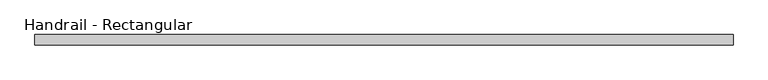
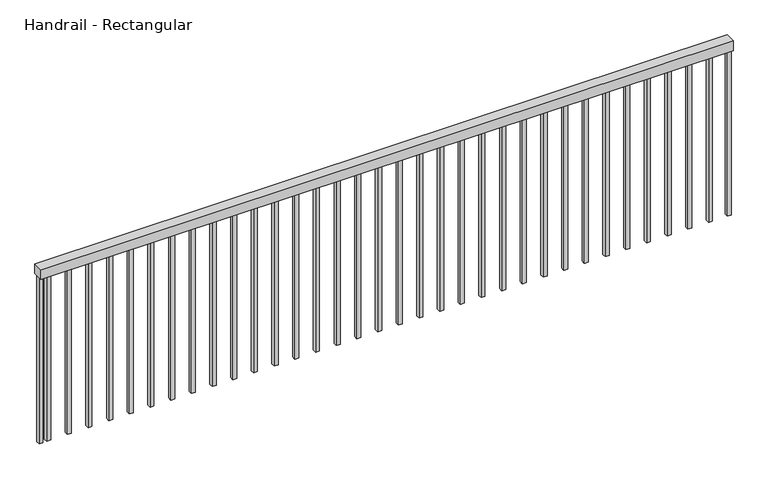
"""IFC4 building model written with IfcOpenShell, lengths in millimetres: railing geometry, Handrail - Rectangular."""

from ifc_helpers import new_model, si_unit, frame, origin, place, context, project, spatial, polyline, outline, extrude, source, transform, mapped, element, save


def handrail_rectangular_9be391eb(model_context):
    return source(origin(), model_context, "Body", "SweptSolid", [
        extrude(outline(polyline([(-6390.3046217, -592.5812264), (-6390.3046217, -643.3812264), (-9790.3046217, -643.3812264), (-9790.3046217, -592.5812264), (-6390.3046217, -592.5812264)])), frame((0.0, 0.0, 6654.4), z_axis=(0.0, 0.0, 1.0), x_axis=(1.0, 0.0, 0.0)), (0.0, 0.0, 1.0), 50.8),
        extrude(outline(polyline([(-9733.5796217, -608.4562264), (-9733.5796217, -627.5062264), (-9752.6296217, -627.5062264), (-9752.6296217, -608.4562264), (-9733.5796217, -608.4562264)])), frame((0.0, 0.0, 5790.8), z_axis=(0.0, 0.0, 1.0), x_axis=(1.0, 0.0, 0.0)), (0.0, 0.0, 1.0), 863.6),
        extrude(outline(polyline([(-9631.9796217, -608.4562264), (-9631.9796217, -627.5062264), (-9651.0296217, -627.5062264), (-9651.0296217, -608.4562264), (-9631.9796217, -608.4562264)])), frame((0.0, 0.0, 5790.8), z_axis=(0.0, 0.0, 1.0), x_axis=(1.0, 0.0, 0.0)), (0.0, 0.0, 1.0), 863.6),
        extrude(outline(polyline([(-9530.3796217, -608.4562264), (-9530.3796217, -627.5062264), (-9549.4296217, -627.5062264), (-9549.4296217, -608.4562264), (-9530.3796217, -608.4562264)])), frame((0.0, 0.0, 5790.8), z_axis=(0.0, 0.0, 1.0), x_axis=(1.0, 0.0, 0.0)), (0.0, 0.0, 1.0), 863.6),
        extrude(outline(polyline([(-9428.7796217, -608.4562264), (-9428.7796217, -627.5062264), (-9447.8296217, -627.5062264), (-9447.8296217, -608.4562264), (-9428.7796217, -608.4562264)])), frame((0.0, 0.0, 5790.8), z_axis=(0.0, 0.0, 1.0), x_axis=(1.0, 0.0, 0.0)), (0.0, 0.0, 1.0), 863.6),
        extrude(outline(polyline([(-9327.1796217, -608.4562264), (-9327.1796217, -627.5062264), (-9346.2296217, -627.5062264), (-9346.2296217, -608.4562264), (-9327.1796217, -608.4562264)])), frame((0.0, 0.0, 5790.8), z_axis=(0.0, 0.0, 1.0), x_axis=(1.0, 0.0, 0.0)), (0.0, 0.0, 1.0), 863.6),
        extrude(outline(polyline([(-9225.5796217, -608.4562264), (-9225.5796217, -627.5062264), (-9244.6296217, -627.5062264), (-9244.6296217, -608.4562264), (-9225.5796217, -608.4562264)])), frame((0.0, 0.0, 5790.8), z_axis=(0.0, 0.0, 1.0), x_axis=(1.0, 0.0, 0.0)), (0.0, 0.0, 1.0), 863.6),
        extrude(outline(polyline([(-9123.9796217, -608.4562264), (-9123.9796217, -627.5062264), (-9143.0296217, -627.5062264), (-9143.0296217, -608.4562264), (-9123.9796217, -608.4562264)])), frame((0.0, 0.0, 5790.8), z_axis=(0.0, 0.0, 1.0), x_axis=(1.0, 0.0, 0.0)), (0.0, 0.0, 1.0), 863.6),
        extrude(outline(polyline([(-9022.3796217, -608.4562264), (-9022.3796217, -627.5062264), (-9041.4296217, -627.5062264), (-9041.4296217, -608.4562264), (-9022.3796217, -608.4562264)])), frame((0.0, 0.0, 5790.8), z_axis=(0.0, 0.0, 1.0), x_axis=(1.0, 0.0, 0.0)), (0.0, 0.0, 1.0), 863.6),
        extrude(outline(polyline([(-8920.7796217, -608.4562264), (-8920.7796217, -627.5062264), (-8939.8296217, -627.5062264), (-8939.8296217, -608.4562264), (-8920.7796217, -608.4562264)])), frame((0.0, 0.0, 5790.8), z_axis=(0.0, 0.0, 1.0), x_axis=(1.0, 0.0, 0.0)), (0.0, 0.0, 1.0), 863.6),
        extrude(outline(polyline([(-8819.1796217, -608.4562264), (-8819.1796217, -627.5062264), (-8838.2296217, -627.5062264), (-8838.2296217, -608.4562264), (-8819.1796217, -608.4562264)])), frame((0.0, 0.0, 5790.8), z_axis=(0.0, 0.0, 1.0), x_axis=(1.0, 0.0, 0.0)), (0.0, 0.0, 1.0), 863.6),
        extrude(outline(polyline([(-8717.5796217, -608.4562264), (-8717.5796217, -627.5062264), (-8736.6296217, -627.5062264), (-8736.6296217, -608.4562264), (-8717.5796217, -608.4562264)])), frame((0.0, 0.0, 5790.8), z_axis=(0.0, 0.0, 1.0), x_axis=(1.0, 0.0, 0.0)), (0.0, 0.0, 1.0), 863.6),
        extrude(outline(polyline([(-8615.9796217, -608.4562264), (-8615.9796217, -627.5062264), (-8635.0296217, -627.5062264), (-8635.0296217, -608.4562264), (-8615.9796217, -608.4562264)])), frame((0.0, 0.0, 5790.8), z_axis=(0.0, 0.0, 1.0), x_axis=(1.0, 0.0, 0.0)), (0.0, 0.0, 1.0), 863.6),
        extrude(outline(polyline([(-8514.3796217, -608.4562264), (-8514.3796217, -627.5062264), (-8533.4296217, -627.5062264), (-8533.4296217, -608.4562264), (-8514.3796217, -608.4562264)])), frame((0.0, 0.0, 5790.8), z_axis=(0.0, 0.0, 1.0), x_axis=(1.0, 0.0, 0.0)), (0.0, 0.0, 1.0), 863.6),
        extrude(outline(polyline([(-8412.7796217, -608.4562264), (-8412.7796217, -627.5062264), (-8431.8296217, -627.5062264), (-8431.8296217, -608.4562264), (-8412.7796217, -608.4562264)])), frame((0.0, 0.0, 5790.8), z_axis=(0.0, 0.0, 1.0), x_axis=(1.0, 0.0, 0.0)), (0.0, 0.0, 1.0), 863.6),
        extrude(outline(polyline([(-8311.1796217, -608.4562264), (-8311.1796217, -627.5062264), (-8330.2296217, -627.5062264), (-8330.2296217, -608.4562264), (-8311.1796217, -608.4562264)])), frame((0.0, 0.0, 5790.8), z_axis=(0.0, 0.0, 1.0), x_axis=(1.0, 0.0, 0.0)), (0.0, 0.0, 1.0), 863.6),
        extrude(outline(polyline([(-8209.5796217, -608.4562264), (-8209.5796217, -627.5062264), (-8228.6296217, -627.5062264), (-8228.6296217, -608.4562264), (-8209.5796217, -608.4562264)])), frame((0.0, 0.0, 5790.8), z_axis=(0.0, 0.0, 1.0), x_axis=(1.0, 0.0, 0.0)), (0.0, 0.0, 1.0), 863.6),
        extrude(outline(polyline([(-8107.9796217, -608.4562264), (-8107.9796217, -627.5062264), (-8127.0296217, -627.5062264), (-8127.0296217, -608.4562264), (-8107.9796217, -608.4562264)])), frame((0.0, 0.0, 5790.8), z_axis=(0.0, 0.0, 1.0), x_axis=(1.0, 0.0, 0.0)), (0.0, 0.0, 1.0), 863.6),
        extrude(outline(polyline([(-8006.3796217, -608.4562264), (-8006.3796217, -627.5062264), (-8025.4296217, -627.5062264), (-8025.4296217, -608.4562264), (-8006.3796217, -608.4562264)])), frame((0.0, 0.0, 5790.8), z_axis=(0.0, 0.0, 1.0), x_axis=(1.0, 0.0, 0.0)), (0.0, 0.0, 1.0), 863.6),
        extrude(outline(polyline([(-7904.7796217, -608.4562264), (-7904.7796217, -627.5062264), (-7923.8296217, -627.5062264), (-7923.8296217, -608.4562264), (-7904.7796217, -608.4562264)])), frame((0.0, 0.0, 5790.8), z_axis=(0.0, 0.0, 1.0), x_axis=(1.0, 0.0, 0.0)), (0.0, 0.0, 1.0), 863.6),
        extrude(outline(polyline([(-7803.1796217, -608.4562264), (-7803.1796217, -627.5062264), (-7822.2296217, -627.5062264), (-7822.2296217, -608.4562264), (-7803.1796217, -608.4562264)])), frame((0.0, 0.0, 5790.8), z_axis=(0.0, 0.0, 1.0), x_axis=(1.0, 0.0, 0.0)), (0.0, 0.0, 1.0), 863.6),
        extrude(outline(polyline([(-7701.5796217, -608.4562264), (-7701.5796217, -627.5062264), (-7720.6296217, -627.5062264), (-7720.6296217, -608.4562264), (-7701.5796217, -608.4562264)])), frame((0.0, 0.0, 5790.8), z_axis=(0.0, 0.0, 1.0), x_axis=(1.0, 0.0, 0.0)), (0.0, 0.0, 1.0), 863.6),
        extrude(outline(polyline([(-7599.9796217, -608.4562264), (-7599.9796217, -627.5062264), (-7619.0296217, -627.5062264), (-7619.0296217, -608.4562264), (-7599.9796217, -608.4562264)])), frame((0.0, 0.0, 5790.8), z_axis=(0.0, 0.0, 1.0), x_axis=(1.0, 0.0, 0.0)), (0.0, 0.0, 1.0), 863.6),
        extrude(outline(polyline([(-7498.3796217, -608.4562264), (-7498.3796217, -627.5062264), (-7517.4296217, -627.5062264), (-7517.4296217, -608.4562264), (-7498.3796217, -608.4562264)])), frame((0.0, 0.0, 5790.8), z_axis=(0.0, 0.0, 1.0), x_axis=(1.0, 0.0, 0.0)), (0.0, 0.0, 1.0), 863.6),
        extrude(outline(polyline([(-7396.7796217, -608.4562264), (-7396.7796217, -627.5062264), (-7415.8296217, -627.5062264), (-7415.8296217, -608.4562264), (-7396.7796217, -608.4562264)])), frame((0.0, 0.0, 5790.8), z_axis=(0.0, 0.0, 1.0), x_axis=(1.0, 0.0, 0.0)), (0.0, 0.0, 1.0), 863.6),
        extrude(outline(polyline([(-7295.1796217, -608.4562264), (-7295.1796217, -627.5062264), (-7314.2296217, -627.5062264), (-7314.2296217, -608.4562264), (-7295.1796217, -608.4562264)])), frame((0.0, 0.0, 5790.8), z_axis=(0.0, 0.0, 1.0), x_axis=(1.0, 0.0, 0.0)), (0.0, 0.0, 1.0), 863.6),
        extrude(outline(polyline([(-7193.5796217, -608.4562264), (-7193.5796217, -627.5062264), (-7212.6296217, -627.5062264), (-7212.6296217, -608.4562264), (-7193.5796217, -608.4562264)])), frame((0.0, 0.0, 5790.8), z_axis=(0.0, 0.0, 1.0), x_axis=(1.0, 0.0, 0.0)), (0.0, 0.0, 1.0), 863.6),
        extrude(outline(polyline([(-7091.9796217, -608.4562264), (-7091.9796217, -627.5062264), (-7111.0296217, -627.5062264), (-7111.0296217, -608.4562264), (-7091.9796217, -608.4562264)])), frame((0.0, 0.0, 5790.8), z_axis=(0.0, 0.0, 1.0), x_axis=(1.0, 0.0, 0.0)), (0.0, 0.0, 1.0), 863.6),
        extrude(outline(polyline([(-6990.3796217, -608.4562264), (-6990.3796217, -627.5062264), (-7009.4296217, -627.5062264), (-7009.4296217, -608.4562264), (-6990.3796217, -608.4562264)])), frame((0.0, 0.0, 5790.8), z_axis=(0.0, 0.0, 1.0), x_axis=(1.0, 0.0, 0.0)), (0.0, 0.0, 1.0), 863.6),
        extrude(outline(polyline([(-6888.7796217, -608.4562264), (-6888.7796217, -627.5062264), (-6907.8296217, -627.5062264), (-6907.8296217, -608.4562264), (-6888.7796217, -608.4562264)])), frame((0.0, 0.0, 5790.8), z_axis=(0.0, 0.0, 1.0), x_axis=(1.0, 0.0, 0.0)), (0.0, 0.0, 1.0), 863.6),
        extrude(outline(polyline([(-6787.1796217, -608.4562264), (-6787.1796217, -627.5062264), (-6806.2296217, -627.5062264), (-6806.2296217, -608.4562264), (-6787.1796217, -608.4562264)])), frame((0.0, 0.0, 5790.8), z_axis=(0.0, 0.0, 1.0), x_axis=(1.0, 0.0, 0.0)), (0.0, 0.0, 1.0), 863.6),
        extrude(outline(polyline([(-6685.5796217, -608.4562264), (-6685.5796217, -627.5062264), (-6704.6296217, -627.5062264), (-6704.6296217, -608.4562264), (-6685.5796217, -608.4562264)])), frame((0.0, 0.0, 5790.8), z_axis=(0.0, 0.0, 1.0), x_axis=(1.0, 0.0, 0.0)), (0.0, 0.0, 1.0), 863.6),
        extrude(outline(polyline([(-6583.9796217, -608.4562264), (-6583.9796217, -627.5062264), (-6603.0296217, -627.5062264), (-6603.0296217, -608.4562264), (-6583.9796217, -608.4562264)])), frame((0.0, 0.0, 5790.8), z_axis=(0.0, 0.0, 1.0), x_axis=(1.0, 0.0, 0.0)), (0.0, 0.0, 1.0), 863.6),
        extrude(outline(polyline([(-6482.3796217, -608.4562264), (-6482.3796217, -627.5062264), (-6501.4296217, -627.5062264), (-6501.4296217, -608.4562264), (-6482.3796217, -608.4562264)])), frame((0.0, 0.0, 5790.8), z_axis=(0.0, 0.0, 1.0), x_axis=(1.0, 0.0, 0.0)), (0.0, 0.0, 1.0), 863.6),
        extrude(outline(polyline([(-9771.2546217, -608.4562264), (-9771.2546217, -627.5062264), (-9790.3046217, -627.5062264), (-9790.3046217, -608.4562264), (-9771.2546217, -608.4562264)])), frame((0.0, 0.0, 5790.8), z_axis=(0.0, 0.0, 1.0), x_axis=(1.0, 0.0, 0.0)), (0.0, 0.0, 1.0), 863.6),
        extrude(outline(polyline([(-6390.3046217, -608.4562264), (-6390.3046217, -627.5062264), (-6409.3546217, -627.5062264), (-6409.3546217, -608.4562264), (-6390.3046217, -608.4562264)])), frame((0.0, 0.0, 5790.8), z_axis=(0.0, 0.0, 1.0), x_axis=(1.0, 0.0, 0.0)), (0.0, 0.0, 1.0), 863.6),
    ])


if __name__ == "__main__":
    model = new_model("IFC4")
    model_context = context("Model", 3, world=origin())
    ifc_project = project(units=[si_unit("LENGTHUNIT", "METRE", prefix="MILLI")], contexts=[model_context])
    site = spatial("IfcSite", under=ifc_project)
    building = spatial("IfcBuilding", under=site)
    placement = place(None, origin())
    handrail_rectangular_shape = handrail_rectangular_9be391eb(model_context)
    element("IfcRailing", 1, ObjectType="Handrail - Rectangular", at=placement, inside=building, context=model_context, shape_type="MappedRepresentation", body=[
        mapped(handrail_rectangular_shape, transform((0.0, 0.0, 0.0), x_axis=(1.0, 0.0, 0.0), y_axis=(0.0, 1.0, 0.0), z_axis=(0.0, 0.0, 1.0))),
    ])
    save(model, "model.ifc")
